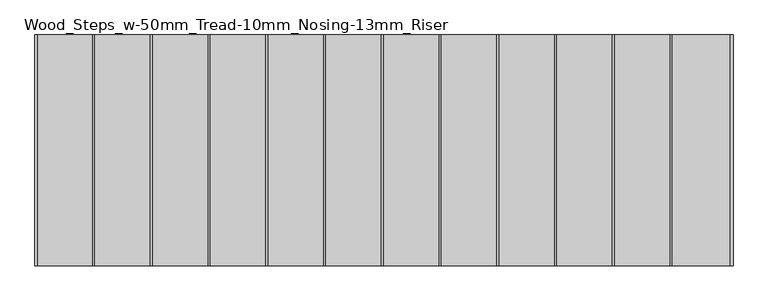
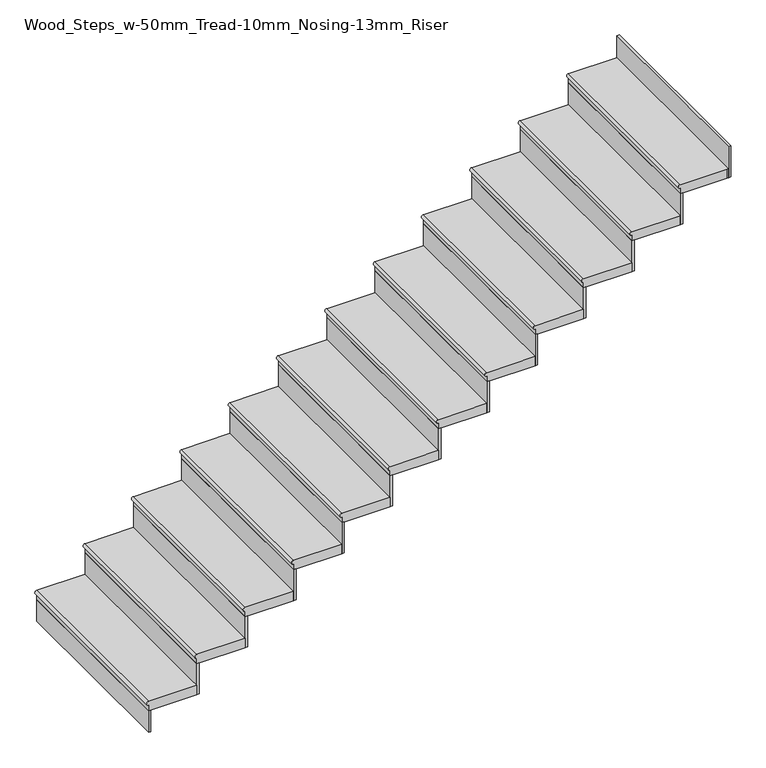
"""IFC4 building model written with IfcOpenShell, lengths in millimetres: stair flight geometry, Wood_Steps_w-50mm_Tread-10mm_Nosing-13mm_Riser."""

from ifc_helpers import new_model, si_unit, frame, origin, place, context, project, spatial, circle_curve, faceted_brep, source, transform, mapped, element, save
from ifc_brep_helpers import plane_surface, cylinder_surface, advanced_brep


def wood_steps_w_50mm_tread_10mm_nosing_13mm_riser_92559dde(model_context):
    return source(origin(), model_context, "Body", "SolidModel", [
        advanced_brep(
        [(-544.509652, 19.7308056, 599.2588235), (-544.509652, 19.7308056, 619.2588235), (-544.509652, 1019.7308056, 619.2588235), (-544.509652, 1019.7308056, 599.2588235), (-294.509652, 1019.7308056, 619.2588235), (-294.509652, 19.7308056, 619.2588235), (-544.509652, 1019.7308056, 569.2588235), (-294.509652, 1019.7308056, 569.2588235), (-294.509652, 19.7308056, 569.2588235), (-544.509652, 19.7308056, 569.2588235)],
        [
            (0, 1, circle_curve(frame((-544.509652, 19.7308056, 609.2588235), z_axis=(0.0, 1.0, 0.0), x_axis=(1.0, 0.0, 0.0)), 10.0)),
            (1, 2),
            (2, 3, circle_curve(frame((-544.509652, 1019.7308056, 609.2588235), z_axis=(0.0, -1.0, 0.0), x_axis=(1.0, 0.0, 0.0)), 10.0)),
            (3, 0),
            (4, 2),
            (1, 5),
            (5, 4),
            (6, 7),
            (7, 8),
            (8, 9),
            (9, 6),
            (4, 7),
            (6, 3),
            (9, 0),
            (8, 5),
        ],
        [
            cylinder_surface(frame((-544.509652, 19.7308056, 609.2588235), z_axis=(0.0, -1.0, 0.0), x_axis=(1.0, 0.0, 0.0)), 10.0),
            plane_surface(frame((-554.509652, 1019.7308056, 619.2588235), z_axis=(0.0, 0.0, 1.0), x_axis=(-1.0, 0.0, 0.0))),
            plane_surface(frame((-554.509652, 1019.7308056, 569.2588235), z_axis=(0.0, 0.0, -1.0), x_axis=(1.0, 0.0, 0.0))),
            plane_surface(frame((-294.509652, 1019.7308056, 619.2588235), z_axis=(0.0, 1.0, 0.0), x_axis=(0.0, 0.0, -1.0))),
            plane_surface(frame((-544.509652, 1019.7308056, 619.2588235), z_axis=(-1.0, 0.0, 0.0), x_axis=(0.0, 0.0, -1.0))),
            plane_surface(frame((-544.509652, 19.7308056, 619.2588235), z_axis=(0.0, -1.0, 0.0), x_axis=(0.0, 0.0, -1.0))),
            plane_surface(frame((-294.509652, 19.7308056, 619.2588235), z_axis=(1.0, 0.0, 0.0), x_axis=(0.0, 0.0, -1.0))),
        ],
        [
            (0, [[1, 2, 3, 4]]),
            (1, [[5, -2, 6, 7]]),
            (2, [[8, 9, 10, 11]]),
            (3, [[-5, 12, -8, 13, -3]]),
            (4, [[-11, 14, -4, -13]]),
            (5, [[-6, -1, -14, -10, 15]]),
            (6, [[-7, -15, -9, -12]]),
        ],
    ),
        faceted_brep([(-544.509652, 19.7308056, 569.2588235), (-544.509652, 19.7308056, 450.0), (-532.009652, 19.7308056, 450.0), (-532.009652, 19.7308056, 569.2588235), (-544.509652, 1019.7308056, 569.2588235), (-532.009652, 1019.7308056, 569.2588235), (-532.009652, 1019.7308056, 450.0), (-544.509652, 1019.7308056, 450.0)], [[[0, 1, 2, 3]], [[4, 5, 6, 7]], [[1, 0, 4, 7]], [[2, 1, 7, 6]], [[3, 2, 6, 5]], [[0, 3, 5, 4]]]),
        faceted_brep([(-294.509652, 19.7308056, 738.5176471), (-294.509652, 19.7308056, 569.2588235), (-282.009652, 19.7308056, 569.2588235), (-282.009652, 19.7308056, 738.5176471), (-294.509652, 1019.7308056, 738.5176471), (-282.009652, 1019.7308056, 738.5176471), (-282.009652, 1019.7308056, 569.2588235), (-294.509652, 1019.7308056, 569.2588235)], [[[0, 1, 2, 3]], [[4, 5, 6, 7]], [[1, 0, 4, 7]], [[2, 1, 7, 6]], [[3, 2, 6, 5]], [[0, 3, 5, 4]]]),
        advanced_brep(
        [(-44.509652, 1019.7308056, 788.5176471), (-294.509652, 1019.7308056, 788.5176471), (-294.509652, 19.7308056, 788.5176471), (-44.509652, 19.7308056, 788.5176471), (-294.509652, 1019.7308056, 738.5176471), (-44.509652, 1019.7308056, 738.5176471), (-44.509652, 19.7308056, 738.5176471), (-294.509652, 19.7308056, 738.5176471), (-294.509652, 1019.7308056, 768.5176471), (-294.509652, 19.7308056, 768.5176471)],
        [
            (0, 1),
            (1, 2),
            (2, 3),
            (3, 0),
            (4, 5),
            (5, 6),
            (6, 7),
            (7, 4),
            (0, 5),
            (4, 8),
            (8, 1, circle_curve(frame((-294.509652, 1019.7308056, 778.5176471), z_axis=(0.0, 1.0, 0.0), x_axis=(1.0, 0.0, 0.0)), 10.0)),
            (7, 9),
            (9, 8),
            (2, 9, circle_curve(frame((-294.509652, 19.7308056, 778.5176471), z_axis=(0.0, -1.0, 0.0), x_axis=(1.0, 0.0, 0.0)), 10.0)),
            (6, 3),
        ],
        [
            plane_surface(frame((-554.509652, 1019.7308056, 788.5176471), z_axis=(0.0, 0.0, 1.0), x_axis=(-1.0, 0.0, 0.0))),
            plane_surface(frame((-554.509652, 1019.7308056, 738.5176471), z_axis=(0.0, 0.0, -1.0), x_axis=(1.0, 0.0, 0.0))),
            plane_surface(frame((-44.509652, 1019.7308056, 788.5176471), z_axis=(0.0, 1.0, 0.0), x_axis=(0.0, 0.0, -1.0))),
            plane_surface(frame((-294.509652, 1019.7308056, 788.5176471), z_axis=(-1.0, 0.0, 0.0), x_axis=(0.0, 0.0, -1.0))),
            plane_surface(frame((-294.509652, 19.7308056, 788.5176471), z_axis=(0.0, -1.0, 0.0), x_axis=(0.0, 0.0, -1.0))),
            plane_surface(frame((-44.509652, 19.7308056, 788.5176471), z_axis=(1.0, 0.0, 0.0), x_axis=(0.0, 0.0, -1.0))),
            cylinder_surface(frame((-294.509652, 19.7308056, 778.5176471), z_axis=(0.0, -1.0, 0.0), x_axis=(1.0, 0.0, 0.0)), 10.0),
        ],
        [
            (0, [[1, 2, 3, 4]]),
            (1, [[5, 6, 7, 8]]),
            (2, [[-1, 9, -5, 10, 11]]),
            (3, [[-8, 12, 13, -10]]),
            (4, [[-3, 14, -12, -7, 15]]),
            (5, [[-4, -15, -6, -9]]),
            (6, [[-14, -2, -11, -13]]),
        ],
    ),
        faceted_brep([(-44.509652, 19.7308056, 907.7764706), (-44.509652, 19.7308056, 738.5176471), (-32.009652, 19.7308056, 738.5176471), (-32.009652, 19.7308056, 907.7764706), (-44.509652, 1019.7308056, 907.7764706), (-32.009652, 1019.7308056, 907.7764706), (-32.009652, 1019.7308056, 738.5176471), (-44.509652, 1019.7308056, 738.5176471)], [[[0, 1, 2, 3]], [[4, 5, 6, 7]], [[1, 0, 4, 7]], [[2, 1, 7, 6]], [[3, 2, 6, 5]], [[0, 3, 5, 4]]]),
        advanced_brep(
        [(205.490348, 1019.7308056, 957.7764706), (-44.509652, 1019.7308056, 957.7764706), (-44.509652, 19.7308056, 957.7764706), (205.490348, 19.7308056, 957.7764706), (-44.509652, 1019.7308056, 907.7764706), (205.490348, 1019.7308056, 907.7764706), (205.490348, 19.7308056, 907.7764706), (-44.509652, 19.7308056, 907.7764706), (-44.509652, 1019.7308056, 937.7764706), (-44.509652, 19.7308056, 937.7764706)],
        [
            (0, 1),
            (1, 2),
            (2, 3),
            (3, 0),
            (4, 5),
            (5, 6),
            (6, 7),
            (7, 4),
            (0, 5),
            (4, 8),
            (8, 1, circle_curve(frame((-44.509652, 1019.7308056, 947.7764706), z_axis=(0.0, 1.0, 0.0), x_axis=(1.0, 0.0, 0.0)), 10.0)),
            (7, 9),
            (9, 8),
            (2, 9, circle_curve(frame((-44.509652, 19.7308056, 947.7764706), z_axis=(0.0, -1.0, 0.0), x_axis=(1.0, 0.0, 0.0)), 10.0)),
            (6, 3),
        ],
        [
            plane_surface(frame((-304.509652, 1019.7308056, 957.7764706), z_axis=(0.0, 0.0, 1.0), x_axis=(-1.0, 0.0, 0.0))),
            plane_surface(frame((-304.509652, 1019.7308056, 907.7764706), z_axis=(0.0, 0.0, -1.0), x_axis=(1.0, 0.0, 0.0))),
            plane_surface(frame((205.490348, 1019.7308056, 957.7764706), z_axis=(0.0, 1.0, 0.0), x_axis=(0.0, 0.0, -1.0))),
            plane_surface(frame((-44.509652, 1019.7308056, 957.7764706), z_axis=(-1.0, 0.0, 0.0), x_axis=(0.0, 0.0, -1.0))),
            plane_surface(frame((-44.509652, 19.7308056, 957.7764706), z_axis=(0.0, -1.0, 0.0), x_axis=(0.0, 0.0, -1.0))),
            plane_surface(frame((205.490348, 19.7308056, 957.7764706), z_axis=(1.0, 0.0, 0.0), x_axis=(0.0, 0.0, -1.0))),
            cylinder_surface(frame((-44.509652, 19.7308056, 947.7764706), z_axis=(0.0, -1.0, 0.0), x_axis=(1.0, 0.0, 0.0)), 10.0),
        ],
        [
            (0, [[1, 2, 3, 4]]),
            (1, [[5, 6, 7, 8]]),
            (2, [[-1, 9, -5, 10, 11]]),
            (3, [[-8, 12, 13, -10]]),
            (4, [[-3, 14, -12, -7, 15]]),
            (5, [[-4, -15, -6, -9]]),
            (6, [[-14, -2, -11, -13]]),
        ],
    ),
        faceted_brep([(205.490348, 19.7308056, 1077.0352941), (205.490348, 19.7308056, 907.7764706), (217.990348, 19.7308056, 907.7764706), (217.990348, 19.7308056, 1077.0352941), (205.490348, 1019.7308056, 1077.0352941), (217.990348, 1019.7308056, 1077.0352941), (217.990348, 1019.7308056, 907.7764706), (205.490348, 1019.7308056, 907.7764706)], [[[0, 1, 2, 3]], [[4, 5, 6, 7]], [[1, 0, 4, 7]], [[2, 1, 7, 6]], [[3, 2, 6, 5]], [[0, 3, 5, 4]]]),
        advanced_brep(
        [(455.490348, 1019.7308056, 1127.0352941), (205.490348, 1019.7308056, 1127.0352941), (205.490348, 19.7308056, 1127.0352941), (455.490348, 19.7308056, 1127.0352941), (205.490348, 1019.7308056, 1077.0352941), (455.490348, 1019.7308056, 1077.0352941), (455.490348, 19.7308056, 1077.0352941), (205.490348, 19.7308056, 1077.0352941), (205.490348, 1019.7308056, 1107.0352941), (205.490348, 19.7308056, 1107.0352941)],
        [
            (0, 1),
            (1, 2),
            (2, 3),
            (3, 0),
            (4, 5),
            (5, 6),
            (6, 7),
            (7, 4),
            (0, 5),
            (4, 8),
            (8, 1, circle_curve(frame((205.490348, 1019.7308056, 1117.0352941), z_axis=(0.0, 1.0, 0.0), x_axis=(1.0, 0.0, 0.0)), 10.0)),
            (7, 9),
            (9, 8),
            (2, 9, circle_curve(frame((205.490348, 19.7308056, 1117.0352941), z_axis=(0.0, -1.0, 0.0), x_axis=(1.0, 0.0, 0.0)), 10.0)),
            (6, 3),
        ],
        [
            plane_surface(frame((-54.509652, 1019.7308056, 1127.0352941), z_axis=(0.0, 0.0, 1.0), x_axis=(-1.0, 0.0, 0.0))),
            plane_surface(frame((-54.509652, 1019.7308056, 1077.0352941), z_axis=(0.0, 0.0, -1.0), x_axis=(1.0, 0.0, 0.0))),
            plane_surface(frame((455.490348, 1019.7308056, 1127.0352941), z_axis=(0.0, 1.0, 0.0), x_axis=(0.0, 0.0, -1.0))),
            plane_surface(frame((205.490348, 1019.7308056, 1127.0352941), z_axis=(-1.0, 0.0, 0.0), x_axis=(0.0, 0.0, -1.0))),
            plane_surface(frame((205.490348, 19.7308056, 1127.0352941), z_axis=(0.0, -1.0, 0.0), x_axis=(0.0, 0.0, -1.0))),
            plane_surface(frame((455.490348, 19.7308056, 1127.0352941), z_axis=(1.0, 0.0, 0.0), x_axis=(0.0, 0.0, -1.0))),
            cylinder_surface(frame((205.490348, 19.7308056, 1117.0352941), z_axis=(0.0, -1.0, 0.0), x_axis=(1.0, 0.0, 0.0)), 10.0),
        ],
        [
            (0, [[1, 2, 3, 4]]),
            (1, [[5, 6, 7, 8]]),
            (2, [[-1, 9, -5, 10, 11]]),
            (3, [[-8, 12, 13, -10]]),
            (4, [[-3, 14, -12, -7, 15]]),
            (5, [[-4, -15, -6, -9]]),
            (6, [[-14, -2, -11, -13]]),
        ],
    ),
        faceted_brep([(455.490348, 19.7308056, 1246.2941176), (455.490348, 19.7308056, 1077.0352941), (467.990348, 19.7308056, 1077.0352941), (467.990348, 19.7308056, 1246.2941176), (455.490348, 1019.7308056, 1246.2941176), (467.990348, 1019.7308056, 1246.2941176), (467.990348, 1019.7308056, 1077.0352941), (455.490348, 1019.7308056, 1077.0352941)], [[[0, 1, 2, 3]], [[4, 5, 6, 7]], [[1, 0, 4, 7]], [[2, 1, 7, 6]], [[3, 2, 6, 5]], [[0, 3, 5, 4]]]),
        advanced_brep(
        [(705.490348, 1019.7308056, 1296.2941176), (455.490348, 1019.7308056, 1296.2941176), (455.490348, 19.7308056, 1296.2941176), (705.490348, 19.7308056, 1296.2941176), (455.490348, 1019.7308056, 1246.2941176), (705.490348, 1019.7308056, 1246.2941176), (705.490348, 19.7308056, 1246.2941176), (455.490348, 19.7308056, 1246.2941176), (455.490348, 1019.7308056, 1276.2941176), (455.490348, 19.7308056, 1276.2941176)],
        [
            (0, 1),
            (1, 2),
            (2, 3),
            (3, 0),
            (4, 5),
            (5, 6),
            (6, 7),
            (7, 4),
            (0, 5),
            (4, 8),
            (8, 1, circle_curve(frame((455.490348, 1019.7308056, 1286.2941176), z_axis=(0.0, 1.0, 0.0), x_axis=(1.0, 0.0, 0.0)), 10.0)),
            (7, 9),
            (9, 8),
            (2, 9, circle_curve(frame((455.490348, 19.7308056, 1286.2941176), z_axis=(0.0, -1.0, 0.0), x_axis=(1.0, 0.0, 0.0)), 10.0)),
            (6, 3),
        ],
        [
            plane_surface(frame((195.490348, 1019.7308056, 1296.2941176), z_axis=(0.0, 0.0, 1.0), x_axis=(-1.0, 0.0, 0.0))),
            plane_surface(frame((195.490348, 1019.7308056, 1246.2941176), z_axis=(0.0, 0.0, -1.0), x_axis=(1.0, 0.0, 0.0))),
            plane_surface(frame((705.490348, 1019.7308056, 1296.2941176), z_axis=(0.0, 1.0, 0.0), x_axis=(0.0, 0.0, -1.0))),
            plane_surface(frame((455.490348, 1019.7308056, 1296.2941176), z_axis=(-1.0, 0.0, 0.0), x_axis=(0.0, 0.0, -1.0))),
            plane_surface(frame((455.490348, 19.7308056, 1296.2941176), z_axis=(0.0, -1.0, 0.0), x_axis=(0.0, 0.0, -1.0))),
            plane_surface(frame((705.490348, 19.7308056, 1296.2941176), z_axis=(1.0, 0.0, 0.0), x_axis=(0.0, 0.0, -1.0))),
            cylinder_surface(frame((455.490348, 19.7308056, 1286.2941176), z_axis=(0.0, -1.0, 0.0), x_axis=(1.0, 0.0, 0.0)), 10.0),
        ],
        [
            (0, [[1, 2, 3, 4]]),
            (1, [[5, 6, 7, 8]]),
            (2, [[-1, 9, -5, 10, 11]]),
            (3, [[-8, 12, 13, -10]]),
            (4, [[-3, 14, -12, -7, 15]]),
            (5, [[-4, -15, -6, -9]]),
            (6, [[-14, -2, -11, -13]]),
        ],
    ),
        faceted_brep([(705.490348, 19.7308056, 1415.5529412), (705.490348, 19.7308056, 1246.2941176), (717.990348, 19.7308056, 1246.2941176), (717.990348, 19.7308056, 1415.5529412), (705.490348, 1019.7308056, 1415.5529412), (717.990348, 1019.7308056, 1415.5529412), (717.990348, 1019.7308056, 1246.2941176), (705.490348, 1019.7308056, 1246.2941176)], [[[0, 1, 2, 3]], [[4, 5, 6, 7]], [[1, 0, 4, 7]], [[2, 1, 7, 6]], [[3, 2, 6, 5]], [[0, 3, 5, 4]]]),
        advanced_brep(
        [(955.490348, 1019.7308056, 1465.5529412), (705.490348, 1019.7308056, 1465.5529412), (705.490348, 19.7308056, 1465.5529412), (955.490348, 19.7308056, 1465.5529412), (705.490348, 1019.7308056, 1415.5529412), (955.490348, 1019.7308056, 1415.5529412), (955.490348, 19.7308056, 1415.5529412), (705.490348, 19.7308056, 1415.5529412), (705.490348, 1019.7308056, 1445.5529412), (705.490348, 19.7308056, 1445.5529412)],
        [
            (0, 1),
            (1, 2),
            (2, 3),
            (3, 0),
            (4, 5),
            (5, 6),
            (6, 7),
            (7, 4),
            (0, 5),
            (4, 8),
            (8, 1, circle_curve(frame((705.490348, 1019.7308056, 1455.5529412), z_axis=(0.0, 1.0, 0.0), x_axis=(1.0, 0.0, 0.0)), 10.0)),
            (7, 9),
            (9, 8),
            (2, 9, circle_curve(frame((705.490348, 19.7308056, 1455.5529412), z_axis=(0.0, -1.0, 0.0), x_axis=(1.0, 0.0, 0.0)), 10.0)),
            (6, 3),
        ],
        [
            plane_surface(frame((445.490348, 1019.7308056, 1465.5529412), z_axis=(0.0, 0.0, 1.0), x_axis=(-1.0, 0.0, 0.0))),
            plane_surface(frame((445.490348, 1019.7308056, 1415.5529412), z_axis=(0.0, 0.0, -1.0), x_axis=(1.0, 0.0, 0.0))),
            plane_surface(frame((955.490348, 1019.7308056, 1465.5529412), z_axis=(0.0, 1.0, 0.0), x_axis=(0.0, 0.0, -1.0))),
            plane_surface(frame((705.490348, 1019.7308056, 1465.5529412), z_axis=(-1.0, 0.0, 0.0), x_axis=(0.0, 0.0, -1.0))),
            plane_surface(frame((705.490348, 19.7308056, 1465.5529412), z_axis=(0.0, -1.0, 0.0), x_axis=(0.0, 0.0, -1.0))),
            plane_surface(frame((955.490348, 19.7308056, 1465.5529412), z_axis=(1.0, 0.0, 0.0), x_axis=(0.0, 0.0, -1.0))),
            cylinder_surface(frame((705.490348, 19.7308056, 1455.5529412), z_axis=(0.0, -1.0, 0.0), x_axis=(1.0, 0.0, 0.0)), 10.0),
        ],
        [
            (0, [[1, 2, 3, 4]]),
            (1, [[5, 6, 7, 8]]),
            (2, [[-1, 9, -5, 10, 11]]),
            (3, [[-8, 12, 13, -10]]),
            (4, [[-3, 14, -12, -7, 15]]),
            (5, [[-4, -15, -6, -9]]),
            (6, [[-14, -2, -11, -13]]),
        ],
    ),
        faceted_brep([(955.490348, 19.7308056, 1584.8117647), (955.490348, 19.7308056, 1415.5529412), (967.990348, 19.7308056, 1415.5529412), (967.990348, 19.7308056, 1584.8117647), (955.490348, 1019.7308056, 1584.8117647), (967.990348, 1019.7308056, 1584.8117647), (967.990348, 1019.7308056, 1415.5529412), (955.490348, 1019.7308056, 1415.5529412)], [[[0, 1, 2, 3]], [[4, 5, 6, 7]], [[1, 0, 4, 7]], [[2, 1, 7, 6]], [[3, 2, 6, 5]], [[0, 3, 5, 4]]]),
        advanced_brep(
        [(1205.490348, 1019.7308056, 1634.8117647), (955.490348, 1019.7308056, 1634.8117647), (955.490348, 19.7308056, 1634.8117647), (1205.490348, 19.7308056, 1634.8117647), (955.490348, 1019.7308056, 1584.8117647), (1205.490348, 1019.7308056, 1584.8117647), (1205.490348, 19.7308056, 1584.8117647), (955.490348, 19.7308056, 1584.8117647), (955.490348, 1019.7308056, 1614.8117647), (955.490348, 19.7308056, 1614.8117647)],
        [
            (0, 1),
            (1, 2),
            (2, 3),
            (3, 0),
            (4, 5),
            (5, 6),
            (6, 7),
            (7, 4),
            (0, 5),
            (4, 8),
            (8, 1, circle_curve(frame((955.490348, 1019.7308056, 1624.8117647), z_axis=(0.0, 1.0, 0.0), x_axis=(1.0, 0.0, 0.0)), 10.0)),
            (7, 9),
            (9, 8),
            (2, 9, circle_curve(frame((955.490348, 19.7308056, 1624.8117647), z_axis=(0.0, -1.0, 0.0), x_axis=(1.0, 0.0, 0.0)), 10.0)),
            (6, 3),
        ],
        [
            plane_surface(frame((695.490348, 1019.7308056, 1634.8117647), z_axis=(0.0, 0.0, 1.0), x_axis=(-1.0, 0.0, 0.0))),
            plane_surface(frame((695.490348, 1019.7308056, 1584.8117647), z_axis=(0.0, 0.0, -1.0), x_axis=(1.0, 0.0, 0.0))),
            plane_surface(frame((1205.490348, 1019.7308056, 1634.8117647), z_axis=(0.0, 1.0, 0.0), x_axis=(0.0, 0.0, -1.0))),
            plane_surface(frame((955.490348, 1019.7308056, 1634.8117647), z_axis=(-1.0, 0.0, 0.0), x_axis=(0.0, 0.0, -1.0))),
            plane_surface(frame((955.490348, 19.7308056, 1634.8117647), z_axis=(0.0, -1.0, 0.0), x_axis=(0.0, 0.0, -1.0))),
            plane_surface(frame((1205.490348, 19.7308056, 1634.8117647), z_axis=(1.0, 0.0, 0.0), x_axis=(0.0, 0.0, -1.0))),
            cylinder_surface(frame((955.490348, 19.7308056, 1624.8117647), z_axis=(0.0, -1.0, 0.0), x_axis=(1.0, 0.0, 0.0)), 10.0),
        ],
        [
            (0, [[1, 2, 3, 4]]),
            (1, [[5, 6, 7, 8]]),
            (2, [[-1, 9, -5, 10, 11]]),
            (3, [[-8, 12, 13, -10]]),
            (4, [[-3, 14, -12, -7, 15]]),
            (5, [[-4, -15, -6, -9]]),
            (6, [[-14, -2, -11, -13]]),
        ],
    ),
        faceted_brep([(1205.490348, 19.7308056, 1754.0705882), (1205.490348, 19.7308056, 1584.8117647), (1217.990348, 19.7308056, 1584.8117647), (1217.990348, 19.7308056, 1754.0705882), (1205.490348, 1019.7308056, 1754.0705882), (1217.990348, 1019.7308056, 1754.0705882), (1217.990348, 1019.7308056, 1584.8117647), (1205.490348, 1019.7308056, 1584.8117647)], [[[0, 1, 2, 3]], [[4, 5, 6, 7]], [[1, 0, 4, 7]], [[2, 1, 7, 6]], [[3, 2, 6, 5]], [[0, 3, 5, 4]]]),
        advanced_brep(
        [(1455.490348, 1019.7308056, 1804.0705882), (1205.490348, 1019.7308056, 1804.0705882), (1205.490348, 19.7308056, 1804.0705882), (1455.490348, 19.7308056, 1804.0705882), (1205.490348, 1019.7308056, 1754.0705882), (1455.490348, 1019.7308056, 1754.0705882), (1455.490348, 19.7308056, 1754.0705882), (1205.490348, 19.7308056, 1754.0705882), (1205.490348, 1019.7308056, 1784.0705882), (1205.490348, 19.7308056, 1784.0705882)],
        [
            (0, 1),
            (1, 2),
            (2, 3),
            (3, 0),
            (4, 5),
            (5, 6),
            (6, 7),
            (7, 4),
            (0, 5),
            (4, 8),
            (8, 1, circle_curve(frame((1205.490348, 1019.7308056, 1794.0705882), z_axis=(0.0, 1.0, 0.0), x_axis=(1.0, 0.0, 0.0)), 10.0)),
            (7, 9),
            (9, 8),
            (2, 9, circle_curve(frame((1205.490348, 19.7308056, 1794.0705882), z_axis=(0.0, -1.0, 0.0), x_axis=(1.0, 0.0, 0.0)), 10.0)),
            (6, 3),
        ],
        [
            plane_surface(frame((945.490348, 1019.7308056, 1804.0705882), z_axis=(0.0, 0.0, 1.0), x_axis=(-1.0, 0.0, 0.0))),
            plane_surface(frame((945.490348, 1019.7308056, 1754.0705882), z_axis=(0.0, 0.0, -1.0), x_axis=(1.0, 0.0, 0.0))),
            plane_surface(frame((1455.490348, 1019.7308056, 1804.0705882), z_axis=(0.0, 1.0, 0.0), x_axis=(0.0, 0.0, -1.0))),
            plane_surface(frame((1205.490348, 1019.7308056, 1804.0705882), z_axis=(-1.0, 0.0, 0.0), x_axis=(0.0, 0.0, -1.0))),
            plane_surface(frame((1205.490348, 19.7308056, 1804.0705882), z_axis=(0.0, -1.0, 0.0), x_axis=(0.0, 0.0, -1.0))),
            plane_surface(frame((1455.490348, 19.7308056, 1804.0705882), z_axis=(1.0, 0.0, 0.0), x_axis=(0.0, 0.0, -1.0))),
            cylinder_surface(frame((1205.490348, 19.7308056, 1794.0705882), z_axis=(0.0, -1.0, 0.0), x_axis=(1.0, 0.0, 0.0)), 10.0),
        ],
        [
            (0, [[1, 2, 3, 4]]),
            (1, [[5, 6, 7, 8]]),
            (2, [[-1, 9, -5, 10, 11]]),
            (3, [[-8, 12, 13, -10]]),
            (4, [[-3, 14, -12, -7, 15]]),
            (5, [[-4, -15, -6, -9]]),
            (6, [[-14, -2, -11, -13]]),
        ],
    ),
        faceted_brep([(1455.490348, 19.7308056, 1923.3294118), (1455.490348, 19.7308056, 1754.0705882), (1467.990348, 19.7308056, 1754.0705882), (1467.990348, 19.7308056, 1923.3294118), (1455.490348, 1019.7308056, 1923.3294118), (1467.990348, 1019.7308056, 1923.3294118), (1467.990348, 1019.7308056, 1754.0705882), (1455.490348, 1019.7308056, 1754.0705882)], [[[0, 1, 2, 3]], [[4, 5, 6, 7]], [[1, 0, 4, 7]], [[2, 1, 7, 6]], [[3, 2, 6, 5]], [[0, 3, 5, 4]]]),
        advanced_brep(
        [(1705.490348, 1019.7308056, 1973.3294118), (1455.490348, 1019.7308056, 1973.3294118), (1455.490348, 19.7308056, 1973.3294118), (1705.490348, 19.7308056, 1973.3294118), (1455.490348, 1019.7308056, 1923.3294118), (1705.490348, 1019.7308056, 1923.3294118), (1705.490348, 19.7308056, 1923.3294118), (1455.490348, 19.7308056, 1923.3294118), (1455.490348, 1019.7308056, 1953.3294118), (1455.490348, 19.7308056, 1953.3294118)],
        [
            (0, 1),
            (1, 2),
            (2, 3),
            (3, 0),
            (4, 5),
            (5, 6),
            (6, 7),
            (7, 4),
            (0, 5),
            (4, 8),
            (8, 1, circle_curve(frame((1455.490348, 1019.7308056, 1963.3294118), z_axis=(0.0, 1.0, 0.0), x_axis=(1.0, 0.0, 0.0)), 10.0)),
            (7, 9),
            (9, 8),
            (2, 9, circle_curve(frame((1455.490348, 19.7308056, 1963.3294118), z_axis=(0.0, -1.0, 0.0), x_axis=(1.0, 0.0, 0.0)), 10.0)),
            (6, 3),
        ],
        [
            plane_surface(frame((1195.490348, 1019.7308056, 1973.3294118), z_axis=(0.0, 0.0, 1.0), x_axis=(-1.0, 0.0, 0.0))),
            plane_surface(frame((1195.490348, 1019.7308056, 1923.3294118), z_axis=(0.0, 0.0, -1.0), x_axis=(1.0, 0.0, 0.0))),
            plane_surface(frame((1705.490348, 1019.7308056, 1973.3294118), z_axis=(0.0, 1.0, 0.0), x_axis=(0.0, 0.0, -1.0))),
            plane_surface(frame((1455.490348, 1019.7308056, 1973.3294118), z_axis=(-1.0, 0.0, 0.0), x_axis=(0.0, 0.0, -1.0))),
            plane_surface(frame((1455.490348, 19.7308056, 1973.3294118), z_axis=(0.0, -1.0, 0.0), x_axis=(0.0, 0.0, -1.0))),
            plane_surface(frame((1705.490348, 19.7308056, 1973.3294118), z_axis=(1.0, 0.0, 0.0), x_axis=(0.0, 0.0, -1.0))),
            cylinder_surface(frame((1455.490348, 19.7308056, 1963.3294118), z_axis=(0.0, -1.0, 0.0), x_axis=(1.0, 0.0, 0.0)), 10.0),
        ],
        [
            (0, [[1, 2, 3, 4]]),
            (1, [[5, 6, 7, 8]]),
            (2, [[-1, 9, -5, 10, 11]]),
            (3, [[-8, 12, 13, -10]]),
            (4, [[-3, 14, -12, -7, 15]]),
            (5, [[-4, -15, -6, -9]]),
            (6, [[-14, -2, -11, -13]]),
        ],
    ),
        faceted_brep([(1705.490348, 19.7308056, 2092.5882353), (1705.490348, 19.7308056, 1923.3294118), (1717.990348, 19.7308056, 1923.3294118), (1717.990348, 19.7308056, 2092.5882353), (1705.490348, 1019.7308056, 2092.5882353), (1717.990348, 1019.7308056, 2092.5882353), (1717.990348, 1019.7308056, 1923.3294118), (1705.490348, 1019.7308056, 1923.3294118)], [[[0, 1, 2, 3]], [[4, 5, 6, 7]], [[1, 0, 4, 7]], [[2, 1, 7, 6]], [[3, 2, 6, 5]], [[0, 3, 5, 4]]]),
        advanced_brep(
        [(1955.490348, 1019.7308056, 2142.5882353), (1705.490348, 1019.7308056, 2142.5882353), (1705.490348, 19.7308056, 2142.5882353), (1955.490348, 19.7308056, 2142.5882353), (1705.490348, 1019.7308056, 2092.5882353), (1955.490348, 1019.7308056, 2092.5882353), (1955.490348, 19.7308056, 2092.5882353), (1705.490348, 19.7308056, 2092.5882353), (1705.490348, 1019.7308056, 2122.5882353), (1705.490348, 19.7308056, 2122.5882353)],
        [
            (0, 1),
            (1, 2),
            (2, 3),
            (3, 0),
            (4, 5),
            (5, 6),
            (6, 7),
            (7, 4),
            (0, 5),
            (4, 8),
            (8, 1, circle_curve(frame((1705.490348, 1019.7308056, 2132.5882353), z_axis=(0.0, 1.0, 0.0), x_axis=(1.0, 0.0, 0.0)), 10.0)),
            (7, 9),
            (9, 8),
            (2, 9, circle_curve(frame((1705.490348, 19.7308056, 2132.5882353), z_axis=(0.0, -1.0, 0.0), x_axis=(1.0, 0.0, 0.0)), 10.0)),
            (6, 3),
        ],
        [
            plane_surface(frame((1445.490348, 1019.7308056, 2142.5882353), z_axis=(0.0, 0.0, 1.0), x_axis=(-1.0, 0.0, 0.0))),
            plane_surface(frame((1445.490348, 1019.7308056, 2092.5882353), z_axis=(0.0, 0.0, -1.0), x_axis=(1.0, 0.0, 0.0))),
            plane_surface(frame((1955.490348, 1019.7308056, 2142.5882353), z_axis=(0.0, 1.0, 0.0), x_axis=(0.0, 0.0, -1.0))),
            plane_surface(frame((1705.490348, 1019.7308056, 2142.5882353), z_axis=(-1.0, 0.0, 0.0), x_axis=(0.0, 0.0, -1.0))),
            plane_surface(frame((1705.490348, 19.7308056, 2142.5882353), z_axis=(0.0, -1.0, 0.0), x_axis=(0.0, 0.0, -1.0))),
            plane_surface(frame((1955.490348, 19.7308056, 2142.5882353), z_axis=(1.0, 0.0, 0.0), x_axis=(0.0, 0.0, -1.0))),
            cylinder_surface(frame((1705.490348, 19.7308056, 2132.5882353), z_axis=(0.0, -1.0, 0.0), x_axis=(1.0, 0.0, 0.0)), 10.0),
        ],
        [
            (0, [[1, 2, 3, 4]]),
            (1, [[5, 6, 7, 8]]),
            (2, [[-1, 9, -5, 10, 11]]),
            (3, [[-8, 12, 13, -10]]),
            (4, [[-3, 14, -12, -7, 15]]),
            (5, [[-4, -15, -6, -9]]),
            (6, [[-14, -2, -11, -13]]),
        ],
    ),
        faceted_brep([(1955.490348, 19.7308056, 2261.8470588), (1955.490348, 19.7308056, 2092.5882353), (1967.990348, 19.7308056, 2092.5882353), (1967.990348, 19.7308056, 2261.8470588), (1955.490348, 1019.7308056, 2261.8470588), (1967.990348, 1019.7308056, 2261.8470588), (1967.990348, 1019.7308056, 2092.5882353), (1955.490348, 1019.7308056, 2092.5882353)], [[[0, 1, 2, 3]], [[4, 5, 6, 7]], [[1, 0, 4, 7]], [[2, 1, 7, 6]], [[3, 2, 6, 5]], [[0, 3, 5, 4]]]),
        advanced_brep(
        [(2205.490348, 1019.7308056, 2311.8470588), (1955.490348, 1019.7308056, 2311.8470588), (1955.490348, 19.7308056, 2311.8470588), (2205.490348, 19.7308056, 2311.8470588), (1955.490348, 1019.7308056, 2261.8470588), (2205.490348, 1019.7308056, 2261.8470588), (2205.490348, 19.7308056, 2261.8470588), (1955.490348, 19.7308056, 2261.8470588), (1955.490348, 1019.7308056, 2291.8470588), (1955.490348, 19.7308056, 2291.8470588)],
        [
            (0, 1),
            (1, 2),
            (2, 3),
            (3, 0),
            (4, 5),
            (5, 6),
            (6, 7),
            (7, 4),
            (0, 5),
            (4, 8),
            (8, 1, circle_curve(frame((1955.490348, 1019.7308056, 2301.8470588), z_axis=(0.0, 1.0, 0.0), x_axis=(1.0, 0.0, 0.0)), 10.0)),
            (7, 9),
            (9, 8),
            (2, 9, circle_curve(frame((1955.490348, 19.7308056, 2301.8470588), z_axis=(0.0, -1.0, 0.0), x_axis=(1.0, 0.0, 0.0)), 10.0)),
            (6, 3),
        ],
        [
            plane_surface(frame((1695.490348, 1019.7308056, 2311.8470588), z_axis=(0.0, 0.0, 1.0), x_axis=(-1.0, 0.0, 0.0))),
            plane_surface(frame((1695.490348, 1019.7308056, 2261.8470588), z_axis=(0.0, 0.0, -1.0), x_axis=(1.0, 0.0, 0.0))),
            plane_surface(frame((2205.490348, 1019.7308056, 2311.8470588), z_axis=(0.0, 1.0, 0.0), x_axis=(0.0, 0.0, -1.0))),
            plane_surface(frame((1955.490348, 1019.7308056, 2311.8470588), z_axis=(-1.0, 0.0, 0.0), x_axis=(0.0, 0.0, -1.0))),
            plane_surface(frame((1955.490348, 19.7308056, 2311.8470588), z_axis=(0.0, -1.0, 0.0), x_axis=(0.0, 0.0, -1.0))),
            plane_surface(frame((2205.490348, 19.7308056, 2311.8470588), z_axis=(1.0, 0.0, 0.0), x_axis=(0.0, 0.0, -1.0))),
            cylinder_surface(frame((1955.490348, 19.7308056, 2301.8470588), z_axis=(0.0, -1.0, 0.0), x_axis=(1.0, 0.0, 0.0)), 10.0),
        ],
        [
            (0, [[1, 2, 3, 4]]),
            (1, [[5, 6, 7, 8]]),
            (2, [[-1, 9, -5, 10, 11]]),
            (3, [[-8, 12, 13, -10]]),
            (4, [[-3, 14, -12, -7, 15]]),
            (5, [[-4, -15, -6, -9]]),
            (6, [[-14, -2, -11, -13]]),
        ],
    ),
        faceted_brep([(2455.490348, 19.7308056, 2600.3647059), (2455.490348, 19.7308056, 2431.1058824), (2467.990348, 19.7308056, 2431.1058824), (2467.990348, 19.7308056, 2600.3647059), (2455.490348, 1019.7308056, 2600.3647059), (2467.990348, 1019.7308056, 2600.3647059), (2467.990348, 1019.7308056, 2431.1058824), (2455.490348, 1019.7308056, 2431.1058824)], [[[0, 1, 2, 3]], [[4, 5, 6, 7]], [[1, 0, 4, 7]], [[2, 1, 7, 6]], [[3, 2, 6, 5]], [[0, 3, 5, 4]]]),
        faceted_brep([(2205.490348, 19.7308056, 2431.1058824), (2205.490348, 19.7308056, 2261.8470588), (2217.990348, 19.7308056, 2261.8470588), (2217.990348, 19.7308056, 2431.1058824), (2205.490348, 1019.7308056, 2431.1058824), (2217.990348, 1019.7308056, 2431.1058824), (2217.990348, 1019.7308056, 2261.8470588), (2205.490348, 1019.7308056, 2261.8470588)], [[[0, 1, 2, 3]], [[4, 5, 6, 7]], [[1, 0, 4, 7]], [[2, 1, 7, 6]], [[3, 2, 6, 5]], [[0, 3, 5, 4]]]),
        advanced_brep(
        [(2455.490348, 1019.7308056, 2481.1058824), (2205.490348, 1019.7308056, 2481.1058824), (2205.490348, 19.7308056, 2481.1058824), (2445.490348, 19.7308056, 2481.1058824), (2455.490348, 19.7308056, 2481.1058824), (2205.490348, 1019.7308056, 2431.1058824), (2455.490348, 1019.7308056, 2431.1058824), (2455.490348, 19.7308056, 2431.1058824), (2445.490348, 19.7308056, 2431.1058824), (2205.490348, 19.7308056, 2431.1058824), (2205.490348, 1019.7308056, 2461.1058824), (2205.490348, 19.7308056, 2461.1058824)],
        [
            (0, 1),
            (1, 2),
            (2, 3),
            (3, 4),
            (4, 0),
            (5, 6),
            (6, 7),
            (7, 8),
            (8, 9),
            (9, 5),
            (0, 6),
            (5, 10),
            (10, 1, circle_curve(frame((2205.490348, 1019.7308056, 2471.1058824), z_axis=(0.0, 1.0, 0.0), x_axis=(1.0, 0.0, 0.0)), 10.0)),
            (9, 11),
            (11, 10),
            (2, 11, circle_curve(frame((2205.490348, 19.7308056, 2471.1058824), z_axis=(0.0, -1.0, 0.0), x_axis=(1.0, 0.0, 0.0)), 10.0)),
            (8, 3),
            (7, 4),
        ],
        [
            plane_surface(frame((-554.509652, 1019.7308056, 2481.1058824), z_axis=(0.0, 0.0, 1.0), x_axis=(-1.0, 0.0, 0.0))),
            plane_surface(frame((-554.509652, 1019.7308056, 2431.1058824), z_axis=(0.0, 0.0, -1.0), x_axis=(1.0, 0.0, 0.0))),
            plane_surface(frame((2455.490348, 1019.7308056, 2481.1058824), z_axis=(0.0, 1.0, 0.0), x_axis=(0.0, 0.0, -1.0))),
            plane_surface(frame((2205.490348, 1019.7308056, 2481.1058824), z_axis=(-1.0, 0.0, 0.0), x_axis=(0.0, 0.0, -1.0))),
            plane_surface(frame((2205.490348, 19.7308056, 2481.1058824), z_axis=(0.0, -1.0, 0.0), x_axis=(0.0, 0.0, -1.0))),
            plane_surface(frame((2445.490348, 19.7308056, 2481.1058824), z_axis=(0.0, -1.0, 0.0), x_axis=(0.0, 0.0, -1.0))),
            plane_surface(frame((2455.490348, 19.7308056, 2481.1058824), z_axis=(1.0, 0.0, 0.0), x_axis=(0.0, 0.0, -1.0))),
            cylinder_surface(frame((2205.490348, 19.7308056, 2471.1058824), z_axis=(0.0, -1.0, 0.0), x_axis=(1.0, 0.0, 0.0)), 10.0),
        ],
        [
            (0, [[1, 2, 3, 4, 5]]),
            (1, [[6, 7, 8, 9, 10]]),
            (2, [[-1, 11, -6, 12, 13]]),
            (3, [[-10, 14, 15, -12]]),
            (4, [[-3, 16, -14, -9, 17]]),
            (5, [[-4, -17, -8, 18]]),
            (6, [[-5, -18, -7, -11]]),
            (7, [[-16, -2, -13, -15]]),
        ],
    ),
    ])


if __name__ == "__main__":
    model = new_model("IFC4")
    model_context = context("Model", 3, world=origin())
    ifc_project = project(units=[si_unit("LENGTHUNIT", "METRE", prefix="MILLI")], contexts=[model_context])
    site = spatial("IfcSite", under=ifc_project)
    building = spatial("IfcBuilding", under=site)
    placement = place(None, origin())
    wood_steps_w_50mm_tread_10mm_nosing_13mm_riser_shape = wood_steps_w_50mm_tread_10mm_nosing_13mm_riser_92559dde(model_context)
    element("IfcStairFlight", 1, ObjectType="Wood_Steps_w-50mm_Tread-10mm_Nosing-13mm_Riser", at=placement, inside=building, context=model_context, shape_type="MappedRepresentation", body=[
        mapped(wood_steps_w_50mm_tread_10mm_nosing_13mm_riser_shape, transform((0.0, 0.0, 0.0), x_axis=(1.0, 0.0, 0.0), y_axis=(0.0, 1.0, 0.0), z_axis=(0.0, 0.0, 1.0))),
    ])
    save(model, "model.ifc")

# Revit data of these elements
# Element 1 (IfcStairFlight, "Wood_Steps_w-50mm_Tread-10mm_Nosing-13mm_Riser")
#   Materials on its faces: "Oak Flooring"
# Materials
#   "Oak Flooring": class "Wood", colour RGB 212 179 113, transparency 0, Description = "Quercus Rubra", Cost = 0
